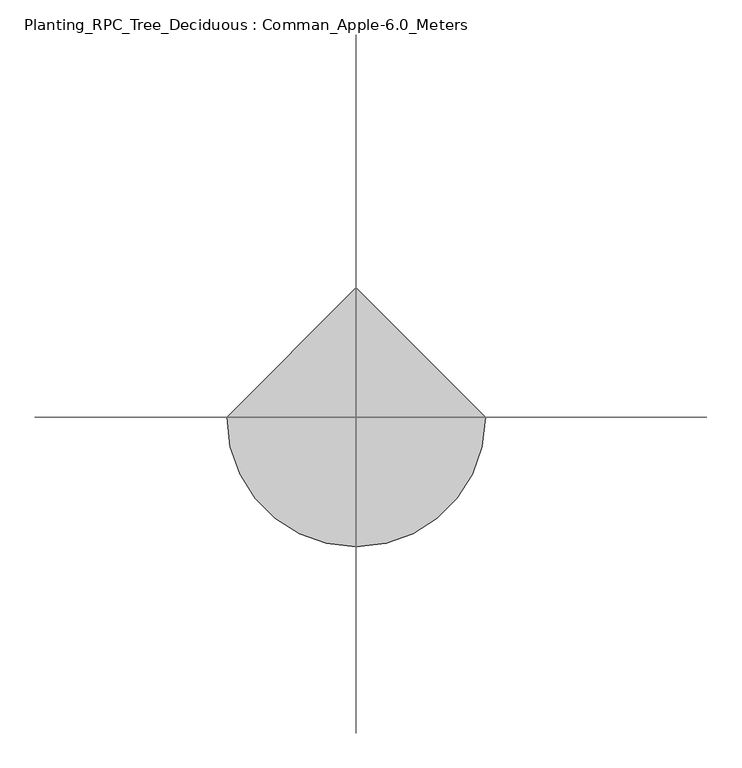
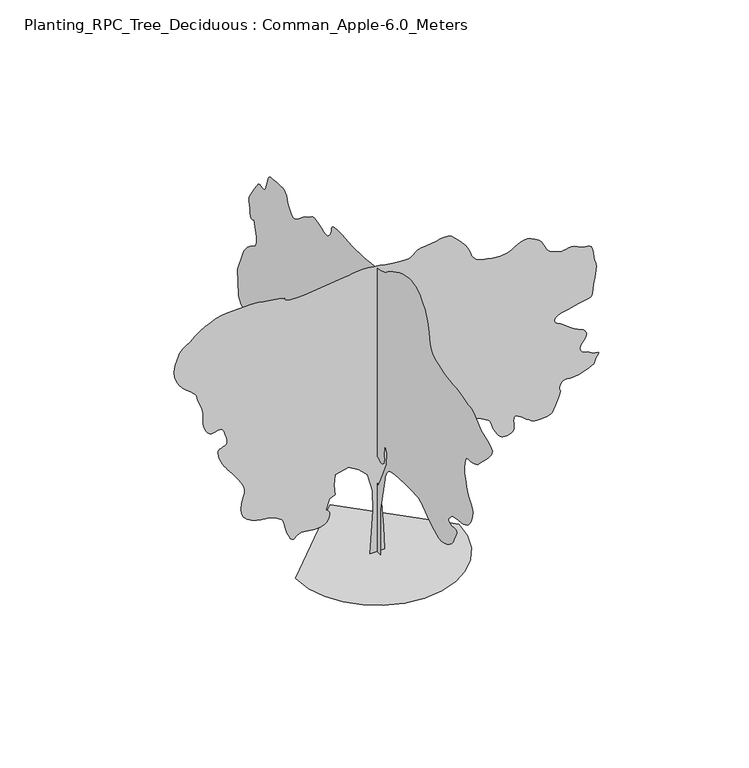
"""IFC4 building model written with IfcOpenShell, lengths in millimetres: geographic element geometry, Planting_RPC_Tree_Deciduous : Comman_Apple-6.0_Meters."""

from ifc_helpers import new_model, si_unit, origin, place, context, project, spatial, triangles, source, transform, mapped, element, save


def planting_rpc_tree_deciduous_comman_apple_6_0_meters_a7a636f8(model_context):
    return source(origin(), model_context, "Body", "Tessellation", [
        triangles([(-6.51e-05, -105.0228319, 0.0074776), (-6.15e-05, 138.9131143, 0.0074703), (-4.84e-05, 99.8833291, 458.6078719), (-3.14e-05, 129.1556067, 1014.7807915), (-1.8e-05, 226.7299288, 1414.8361691), (-8.5e-06, 392.6053236, 1649.0138809), (-1.1e-06, 577.9979682, 1805.1340027), (2.6e-06, 753.6305981, 1844.161417), (3.5e-06, 948.7807503, 1775.8613708), (1.5e-06, 1007.3257959, 1678.2863674), (-4e-06, 890.2357046, 1551.4387321), (-8.4e-06, 929.2657351, 1385.5635372), (-1.44e-05, 1153.685903, 1073.3258371), (-1.47e-05, 1543.9836639, 868.4182137), (-8.5e-06, 2109.9142365, 790.3606236), (7.6e-06, 2451.4244957, 1161.1408985), (2.53e-05, 2802.702182, 1580.7112186), (3.2e-05, 3349.1025513, 1531.9237896), (3.84e-05, 3544.2528488, 1649.0138809), (4.53e-05, 3534.5028625, 1883.1914474), (4.5e-05, 3358.8778267, 1961.2515083), (4.95e-05, 3232.0277206, 2175.9142776), (5.43e-05, 3534.5028625, 2185.6716763), (5.98e-05, 4139.453437, 2068.584201), (6.19e-05, 4208.0283211, 2104.1717091), (6.39e-05, 4273.9283684, 2140.0141434), (6.59e-05, 4334.553447, 2176.3691917), (6.78e-05, 4387.2284294, 2213.4942513), (6.96e-05, 4429.328476, 2251.6417774), (7.12e-05, 4458.2034576, 2291.0693127), (7.26e-05, 4471.2035362, 2332.0343994), (8.79e-05, 4500.4784935, 2829.6522812), (9.79e-05, 4334.6034439, 3249.2275429), (9.86e-05, 4317.5033249, 3282.3275574), (9.94e-05, 4292.2284142, 3321.5527794), (0.0001002, 4260.1033401, 3364.7027618), (0.000101, 4222.5283081, 3409.5526405), (0.0001017, 4180.8532356, 3453.9028404), (0.0001023, 4136.4533295, 3495.527916), (0.0001027, 4090.6782166, 3532.2027122), (0.0001029, 4046.5782921, 3560.9279938), (0.0001029, 4006.7531067, 3582.8278198), (0.000103, 3971.8782005, 3601.8278229), (0.0001031, 3942.6282417, 3621.8527634), (0.0001036, 3919.7031876, 3646.8529816), (0.0001043, 3903.7779968, 3680.7029503), (0.0001056, 3895.5282097, 3727.3530098), (0.0001072, 3894.4779831, 3782.2781456), (0.0001089, 3899.0529945, 3838.2279282), (0.0001108, 3908.3280098, 3895.0532387), (0.0001127, 3921.3530869, 3952.5282188), (0.0001147, 3937.2032822, 4010.528167), (0.0001167, 3954.9280724, 4068.8783844), (0.0001187, 3973.5780968, 4127.4033005), (0.0001184, 3998.5533165, 4107.2783661), (0.0001184, 4022.8532867, 4091.9531387), (0.0001185, 4045.7783409, 4086.1782005), (0.0001191, 4066.6532295, 4094.7532585), (0.0001202, 4084.8032845, 4122.4283134), (0.0001219, 4099.5532562, 4174.003363), (0.0001245, 4110.1781891, 4254.2534065), (0.000127, 4120.6784203, 4333.2285278), (0.0001287, 4132.0283089, 4385.4035408), (0.0001299, 4139.1281662, 4422.2036201), (0.0001309, 4136.8033081, 4455.0786484), (0.0001318, 4120.0031708, 4495.478508), (0.0001331, 4083.5533607, 4554.8286644), (0.0001348, 4022.3783157, 4644.5537109), (0.0001367, 3956.5782623, 4741.1289207), (0.0001382, 3906.9780922, 4815.003772), (0.0001392, 3869.5280525, 4868.5789902), (0.0001398, 3840.0781059, 4904.2041412), (0.0001401, 3814.5529198, 4924.3290756), (0.0001399, 3788.8780334, 4931.3042313), (0.0001393, 3758.9281174, 4927.5038818), (0.0001386, 3727.67799, 4918.0288788), (0.0001379, 3700.2029228, 4909.0788437), (0.0001374, 3675.45298, 4904.7291092), (0.0001372, 3652.4029335, 4909.0788437), (0.0001374, 3630.0528442, 4926.2289597), (0.000138, 3607.3527763, 4960.2792068), (0.0001393, 3583.2777924, 5015.3287537), (0.0001409, 3562.2279144, 5079.6288986), (0.0001424, 3546.3027237, 5137.7538391), (0.0001437, 3531.0527824, 5188.4042358), (0.0001447, 3512.0527794, 5230.1540131), (0.0001452, 3484.8526955, 5261.6794144), (0.0001452, 3445.0278008, 5281.604361), (0.0001446, 3388.1277855, 5288.5295197), (0.0001436, 3319.3276245, 5291.5793335), (0.0001428, 3248.6275795, 5298.5544891), (0.000142, 3178.9774704, 5306.2040222), (0.0001411, 3113.2274139, 5311.3042923), (0.0001402, 3054.3025223, 5310.5793365), (0.0001392, 3005.1273262, 5300.8293503), (0.000138, 2968.5772316, 5278.778952), (0.0001369, 2944.7272339, 5253.1543533), (0.0001361, 2929.602285, 5232.6294434), (0.0001354, 2919.9272942, 5214.0044174), (0.0001347, 2912.4774582, 5194.003894), (0.0001338, 2904.0023941, 5169.4042328), (0.0001326, 2891.2523003, 5136.9288895), (0.000131, 2871.0023735, 5093.3792221), (0.0001292, 2844.6522377, 5045.379245), (0.0001275, 2815.5772682, 5003.1539154), (0.000126, 2783.4271957, 4968.9542587), (0.0001248, 2747.8773308, 4945.0039764), (0.0001238, 2708.5521149, 4933.504097), (0.0001233, 2665.1521477, 4936.7039017), (0.0001232, 2617.3021614, 4956.7788391), (0.0001234, 2569.6771614, 4988.2542435), (0.0001238, 2525.4769524, 5023.3038483), (0.0001243, 2482.1194244, 5060.7288895), (0.0001247, 2437.0593842, 5099.3538574), (0.0001252, 2387.7318718, 5138.0038239), (0.0001254, 2331.5768692, 5175.4288651), (0.0001255, 2266.0343582, 5210.4790512), (0.0001256, 2205.0142456, 5244.5542969), (0.0001259, 2159.0142918, 5277.6040237), (0.0001262, 2120.3541515, 5306.2290207), (0.0001262, 2081.3542065, 5327.0044968), (0.0001258, 2034.3291698, 5336.5044983), (0.0001247, 1971.6040741, 5331.3292328), (0.0001227, 1885.4940685, 5308.0544907), (0.0001205, 1797.391452, 5276.8540695), (0.0001188, 1730.2863911, 5251.9544266), (0.0001175, 1678.8813892, 5236.1042313), (0.0001168, 1637.8888332, 5232.0288986), (0.0001166, 1602.0163136, 5242.4794235), (0.0001169, 1565.9737461, 5270.1544785), (0.0001177, 1524.4687214, 5317.8044769), (0.0001188, 1490.9861721, 5373.8045471), (0.0001201, 1475.2561729, 5423.9793915), (0.0001212, 1466.3511932, 5467.3296524), (0.0001221, 1453.3511147, 5502.8292297), (0.0001225, 1425.3286972, 5529.4543488), (0.0001222, 1371.366148, 5546.1794907), (0.000121, 1280.5334656, 5551.979718), (0.0001195, 1182.4759335, 5550.8792038), (0.0001183, 1108.9958982, 5547.8793869), (0.0001174, 1052.4133781, 5543.5296524), (0.0001165, 1005.0483187, 5538.3293884), (0.0001156, 959.220738, 5532.7791458), (0.0001147, 907.2482563, 5527.4044739), (0.0001136, 841.4482029, 5522.7041794), (0.0001125, 772.3506037, 5519.7043625), (0.0001115, 711.6155754, 5518.9044113), (0.0001107, 653.2705175, 5520.154335), (0.0001099, 591.3404677, 5523.2791443), (0.000109, 519.8504273, 5528.1294296), (0.0001078, 432.8303392, 5534.5046219), (0.0001065, 324.3052774, 5542.2291504), (0.000105, 203.687658, 5552.8796631), (0.0001037, 86.9965703, 5567.6043457), (0.0001026, -21.8426915, 5585.7544006), (0.0001018, -118.9050968, 5606.6292892), (0.0001012, -200.2644113, 5629.5546341), (0.0001011, -261.9952181, 5653.8543137), (0.0001012, -300.1702317, 5678.8295334), (0.0001016, -342.4727732, 5713.0297714), (0.000102, -413.9603428, 5761.2297363), (0.0001023, -506.7854181, 5817.0798157), (0.0001024, -613.0929554, 5874.3298096), (0.0001023, -725.0330704, 5926.6045258), (0.0001019, -834.75319, 5967.6299286), (0.0001011, -934.4057556, 5991.07966), (0.0001, -1022.9033335, 5999.8047089), (9.88e-05, -1104.7484104, 6000.0046967), (9.74e-05, -1180.4459702, 5990.3047073), (9.57e-05, -1250.5110249, 5969.3298248), (9.38e-05, -1315.4560432, 5935.7295502), (9.14e-05, -1375.7936394, 5888.1545471), (8.87e-05, -1432.0336658, 5825.2049011), (8.63e-05, -1478.7161362, 5768.8048553), (8.48e-05, -1512.7687088, 5733.7546692), (8.36e-05, -1538.2837212, 5707.9295013), (8.25e-05, -1559.3636845, 5679.2045105), (8.09e-05, -1580.1012268, 5635.454274), (7.84e-05, -1604.5962433, 5564.5545319), (7.46e-05, -1636.941362, 5454.4042786), (7.05e-05, -1667.1512913, 5330.3292938), (6.7e-05, -1688.656374, 5223.97939), (6.39e-05, -1710.6739254, 5132.8541382), (6.11e-05, -1742.4214062, 5054.3292801), (5.83e-05, -1793.1164223, 4985.8788071), (5.53e-05, -1871.9714928, 4924.9540375), (5.19e-05, -1988.2065491, 4868.9789658), (4.87e-05, -2119.0091755, 4825.5040031), (4.62e-05, -2237.6917568, 4799.6038399), (4.41e-05, -2347.6668755, 4784.9788605), (4.22e-05, -2452.3543808, 4775.3288681), (4.04e-05, -2555.1521759, 4764.2786705), (3.83e-05, -2659.5022018, 4745.5539413), (3.57e-05, -2768.8022163, 4712.8539024), (3.33e-05, -2866.4523605, 4683.5786545), (3.19e-05, -2939.5522591, 4672.2287659), (3.09e-05, -2996.927536, 4668.05373), (2.99e-05, -3047.4773575, 4660.2786232), (2.85e-05, -3100.0773445, 4638.1788094), (2.61e-05, -3163.6025368, 4590.9787834), (2.24e-05, -3246.9276833, 4507.9536186), (1.83e-05, -3354.9527756, 4422.0536293), (1.48e-05, -3474.4277504, 4364.503363), (1.18e-05, -3586.9278603, 4321.8033531), (9.3e-06, -3673.9780701, 4280.47855), (7e-06, -3717.153051, 4227.0283241), (5e-06, -3698.0280556, 4147.9782074), (2.9e-06, -3598.177755, 4029.8281517), (1.1e-06, -3473.4528099, 3906.2781349), (-3e-07, -3385.2276718, 3815.6781418), (-1.3e-06, -3323.4776619, 3751.5279877), (-1.9e-06, -3278.1025246, 3707.3530678), (-2.2e-06, -3239.0275841, 3676.6529068), (-2.3e-06, -3196.2275803, 3652.9528999), (-2.1e-06, -3139.5775497, 3629.777861), (-1.7e-06, -3075.1774109, 3613.37799), (-9e-07, -3016.2275208, 3608.6029907), (-2e-07, -2963.4272552, 3606.7278145), (2e-07, -2917.4774437, 3599.0529922), (2e-07, -2879.0021759, 3576.8528938), (-7e-07, -2848.7272797, 3531.452758), (-2.7e-06, -2827.3521309, 3454.1278267), (-5.1e-06, -2815.7522575, 3369.9277336), (-7e-06, -2813.3521133, 3305.0276253), (-8.6e-06, -2818.6523712, 3252.4026398), (-1.02e-05, -2830.0772552, 3205.052623), (-1.19e-05, -2846.1271477, 3156.0024193), (-1.39e-05, -2865.2274353, 3098.2524559), (-1.64e-05, -2885.9023361, 3024.8022881), (-1.92e-05, -2914.627327, 2946.6774055), (-2.18e-05, -2954.4522217, 2877.5772629), (-2.43e-05, -2998.5524368, 2814.6273262), (-2.67e-05, -3040.0775185, 2754.9021927), (-2.9e-05, -3072.2275909, 2695.5270378), (-3.11e-05, -3088.152491, 2633.6020386), (-3.3e-05, -3081.052343, 2566.2020828), (-3.46e-05, -3060.4274391, 2500.277037), (-3.6e-05, -3039.1022873, 2443.7194427), (-3.71e-05, -3015.2522896, 2395.18694), (-3.79e-05, -2986.9272743, 2353.3118797), (-3.85e-05, -2952.3273514, 2316.7293743), (-3.88e-05, -2909.5023491, 2284.0717747), (-3.89e-05, -2856.6273788, 2253.9743385), (-3.87e-05, -2791.7272705, 2230.5618141), (-3.8e-05, -2717.452153, 2216.0268002), (-3.71e-05, -2638.7520149, 2206.0967377), (-3.62e-05, -2560.5271385, 2196.5117123), (-3.56e-05, -2487.799601, 2182.9993103), (-3.53e-05, -2425.47201, 2161.2942398), (-3.56e-05, -2378.5043827, 2127.129174), (-3.62e-05, -2345.7043499, 2089.8041267), (-3.68e-05, -2322.8042942, 2060.3341232), (-3.73e-05, -2310.1443111, 2037.0066227), (-3.78e-05, -2308.0692924, 2018.1191128), (-3.84e-05, -2316.9168629, 2001.9616688), (-3.92e-05, -2337.029298, 1986.8265461), (-4.01e-05, -2368.7468388, 1971.0090523), (-4.1e-05, -2411.2468609, 1962.5040482), (-4.16e-05, -2459.0394379, 1965.0915356), (-4.21e-05, -2505.4770103, 1970.754126), (-4.27e-05, -2543.876992, 1971.4641117), (-4.34e-05, -2567.6019974, 1959.2041042), (-4.44e-05, -2569.9771431, 1925.949012), (-4.59e-05, -2544.3769615, 1863.6765049), (-4.75e-05, -2509.7520401, 1792.5014889), (-4.89e-05, -2484.8695473, 1735.1513557), (-4.99e-05, -2462.7095627, 1687.5312973), (-5.08e-05, -2436.2819607, 1645.5437439), (-5.14e-05, -2398.5893486, 1605.0912712), (-5.19e-05, -2342.631863, 1562.0787804), (-5.22e-05, -2261.4142914, 1512.4087017), (-5.2e-05, -2169.1316975, 1473.3237328), (-5.1e-05, -2083.5066914, 1461.3762062), (-4.95e-05, -2002.8290577, 1471.4462311), (-4.76e-05, -1925.3965748, 1498.4137711), (-4.53e-05, -1849.4990273, 1537.1587898), (-4.28e-05, -1773.4289612, 1582.5612511), (-4.02e-05, -1695.4838642, 1629.498793), (-3.77e-05, -1622.0062271, 1676.8063705), (-3.54e-05, -1558.0836754, 1724.7963192), (-3.31e-05, -1500.136195, 1770.5689613), (-3.11e-05, -1444.578685, 1811.2214218), (-2.93e-05, -1387.8260445, 1843.8489361), (-2.77e-05, -1326.2960793, 1865.5564774), (-2.64e-05, -1256.4010723, 1873.4340488), (-2.5e-05, -1159.1384045, 1874.2889385), (-2.3e-05, -1027.910804, 1875.4840691), (-2.07e-05, -877.7382116, 1874.971455), (-1.86e-05, -723.6380974, 1870.7039829), (-1.67e-05, -580.6329818, 1860.6339581), (-1.55e-05, -463.7428782, 1842.7115055), (-1.52e-05, -387.9878002, 1814.8914013), (-1.57e-05, -343.2127716, 1776.8839828), (-1.66e-05, -308.1652379, 1730.6863667), (-1.77e-05, -281.2252217, 1677.6614056), (-1.92e-05, -260.7727092, 1619.1738419), (-2.08e-05, -245.1829449, 1556.5887085), (-2.26e-05, -232.8366782, 1491.2736546), (-2.44e-05, -222.1121693, 1424.5935677), (-3.85e-05, -114.7803395, 897.6907001), (-2.01e-05, -26.9632706, 1297.7460777), (-1.3e-05, -173.3248856, 1609.9838505), (-6.5e-06, -300.1727388, 1892.9489914), (2e-07, -319.6852469, 2127.129174), (4.7e-06, -251.3852008, 2244.2167946), (-4e-07, -222.1119331, 2058.8266571), (-1.7e-06, -228.0859325, 2017.1790539), (-3e-06, -232.2679447, 1976.5565334), (-4.1e-06, -232.865183, 1937.9815624), (-5.1e-06, -228.0859325, 1902.4790783), (-5.9e-06, -216.1379155, 1871.0740185), (-6.4e-06, -195.2293988, 1844.788995), (-6.5e-06, -163.5673779, 1824.6489452), (-6.1e-06, -127.1833524, 1819.4714996), (-5.2e-06, -93.5303284, 1831.0189053), (-4.2e-06, -62.949051, 1849.7389835), (-3.3e-06, -35.7820297, 1866.0664753), (-2.9e-06, -12.3698845, 1870.4490566), (-3.1e-06, 6.9458055, 1853.3239391), (-4.3e-06, 21.8237678, 1805.1340027), (-6.1e-06, 32.3777748, 1741.0688725), (-7.7e-06, 39.3472803, 1682.1263947), (-9.3e-06, 43.330036, 1627.4512436), (-1.08e-05, 44.9230347, 1576.1888203), (-1.22e-05, 44.724037, 1527.4862698), (-1.37e-05, 43.330036, 1480.4911732), (-1.51e-05, 41.3385332, 1434.3511116), (137.391859, 0.0003253, 0.0), (-133.3141101, 0.0003334, 0.0), (-73.1573078, 0.0002372, 832.1731876), (-83.1833128, 0.0002433, 1223.1935062), (-183.4456522, 0.0001982, 1574.1087147), (-333.8377625, 0.0002049, 1724.5014244), (-534.3604428, 0.0002126, 1844.8164642), (-785.015601, 0.0002192, 1784.6589443), (-805.0681561, 0.0002168, 1584.1363003), (-785.015601, 0.0002134, 1393.6386257), (-885.278231, 0.0002156, 1343.5060753), (-955.4607931, 0.0002149, 1153.0084007), (-936.3432827, 0.0002675, 1139.8859459), (-918.5407356, 0.0002668, 1125.3558735), (-903.3707314, 0.0002661, 1108.0233559), (-892.1456898, 0.0002654, 1086.4808481), (-886.1831903, 0.0002648, 1059.3258196), (-886.7981964, 0.0002643, 1025.1533415), (-895.3032005, 0.0002639, 982.565752), (-913.9532249, 0.0002639, 940.0632591), (-942.5982788, 0.0002642, 906.5057144), (-978.963283, 0.0002649, 881.0181713), (-1020.7633478, 0.0002659, 862.7181982), (-1065.71838, 0.0002671, 850.7331739), (-1111.553373, 0.0002683, 844.1856812), (-1155.9834372, 0.0002696, 842.1981571), (-1199.4784567, 0.000271, 844.8881819), (-1243.6759769, 0.0002724, 851.4356747), (-1288.0485592, 0.0002738, 859.5631582), (-1332.0685467, 0.0002752, 866.9856703), (-1375.2135876, 0.0002766, 871.4282043), (-1416.9560978, 0.0002778, 870.610667), (-1456.7686386, 0.0002789, 862.2507122), (-1490.9986713, 0.0002796, 844.3906832), (-1518.2137253, 0.0002801, 821.2681847), (-1541.2187164, 0.0002805, 799.9006662), (-1562.8187061, 0.0002809, 787.3031067), (-1585.8236973, 0.0002817, 790.4881594), (-1613.0387512, 0.0002829, 816.475672), (-1647.2663132, 0.0002313, 872.2782251), (-1679.7413658, 0.0002334, 944.3882858), (-1702.0463997, 0.0002351, 1013.3457773), (-1717.508828, 0.0002365, 1077.2133905), (-1729.4639122, 0.0002377, 1134.0684231), (-1741.2438618, 0.0002387, 1181.9784348), (-1756.1814674, 0.0002397, 1219.0134562), (-1777.6064678, 0.0002407, 1243.2460613), (-1804.2939377, 0.0002418, 1262.5659576), (-1833.963929, 0.000243, 1284.8709915), (-1868.368951, 0.0002444, 1308.2261066), (-1909.2639839, 0.000246, 1330.7035137), (-1958.3990662, 0.0002477, 1350.3761501), (-2017.5341194, 0.0002497, 1365.3136105), (-2088.4191822, 0.0002519, 1373.5860706), (-2170.7616852, 0.0002011, 1382.5010788), (-2258.5417923, 0.000204, 1401.9385551), (-2344.9193687, 0.0002071, 1433.8310852), (-2423.054425, 0.0002101, 1480.1036968), (-2486.1043556, 0.0002129, 1542.6862141), (-2527.2271362, 0.0002153, 1623.5087517), (-2539.6019623, 0.0002172, 1724.5014244), (-2528.5270569, 0.0002183, 1822.2489464), (-2508.6771057, 0.0002189, 1897.5490013), (-2487.2420769, 0.0002192, 1958.6416386), (-2471.4293793, 0.0001661, 2013.7690876), (-2468.4170631, 0.0001669, 2071.1791008), (-2485.3994568, 0.0001684, 2139.1117275), (-2529.5769928, 0.000171, 2225.8093426), (-2588.3771828, 0.0001741, 2318.6767845), (-2644.0269836, 0.000177, 2400.3194756), (-2695.8270195, 0.0001796, 2471.7869156), (-2743.0773331, 0.000182, 2534.1270058), (-2785.0520966, 0.0001306, 2588.4271797), (-2821.0522247, 0.0001324, 2635.6772026), (-2850.4021774, 0.0001339, 2676.9770073), (-2878.5522034, 0.0001354, 2723.8270546), (-2908.6274025, 0.0001372, 2782.7522369), (-2936.4274498, 0.000139, 2847.4523575), (-2957.7523109, 0.0001406, 2911.6522179), (-2968.3522453, 0.0001418, 2969.0024963), (-2964.0525078, 0.0001423, 3013.2024147), (-2940.6524826, 0.000142, 3037.927359), (-2905.0023331, 0.0001411, 3050.052491), (-2869.2021927, 0.0001402, 3062.5523094), (-2836.72714, 0.0001395, 3078.1775185), (-2811.1022507, 0.000139, 3099.7773628), (-2795.8023125, 0.000139, 3130.1525436), (-2794.3771088, 0.0001396, 3172.1025993), (-2810.3022995, 0.0001409, 3228.4276497), (-2831.7271545, 8.9e-05, 3286.3526024), (-2846.6774048, 9.02e-05, 3332.2027107), (-2858.4522675, 9.1e-05, 3367.3276016), (-2870.4024101, 9.18e-05, 3393.1777679), (-2885.8523392, 9.25e-05, 3411.1278351), (-2908.17743, 9.33e-05, 3422.5777176), (-2940.6524826, 9.44e-05, 3428.9526192), (-2978.7524826, 9.55e-05, 3427.0527351), (-3016.0025345, 9.65e-05, 3417.4277412), (-3052.7023293, 9.74e-05, 3407.1277885), (-3089.2524239, 9.85e-05, 3403.1027435), (-3125.9775078, 9.97e-05, 3412.4277557), (-3163.2025612, 0.0001012, 3442.1026886), (-3201.3275597, 0.0001032, 3499.1276962), (-3229.5025841, 0.0001051, 3569.6277534), (-3241.3777313, 0.0001065, 3637.1529922), (-3243.9525742, 0.0001076, 3704.8529297), (-3244.2275574, 0.0001086, 3775.9029533), (-3249.2525414, 5.65e-05, 3853.4031647), (-3266.0276802, 5.83e-05, 3940.5780762), (-3301.5775452, 6.09e-05, 4040.5533691), (-3337.877655, 6.33e-05, 4130.928376), (-3357.5276184, 6.48e-05, 4192.7283829), (-3368.4028267, 6.58e-05, 4234.1784691), (-3378.4027977, 6.65e-05, 4263.5284218), (-3395.4276306, 6.74e-05, 4289.0033203), (-3427.3277184, 6.88e-05, 4318.8785316), (-3482.0528664, 7.1e-05, 4361.3785538), (-3552.8529053, 2.06e-05, 4417.8785934), (-3623.6529442, 2.37e-05, 4484.3786041), (-3688.3030678, 2.68e-05, 4561.0535751), (-3740.6780685, 2.96e-05, 4648.0787865), (-3774.6530296, 3.21e-05, 4745.6289368), (-3784.0780357, 3.4e-05, 4853.8540169), (-3762.7778824, 3.51e-05, 4972.9790131), (-3729.8778557, -1.77e-05, 5076.7040771), (-3704.502951, -1.74e-05, 5145.8539261), (-3680.7029503, -1.74e-05, 5191.3290573), (-3652.5279259, -1.78e-05, 5224.0043884), (-3614.0029518, -1.85e-05, 5254.7792542), (-3559.1778099, -1.95e-05, 5294.454158), (-3482.0528664, -2.09e-05, 5353.9790131), (-3391.1775993, -2.26e-05, 5424.8793365), (-3298.9027084, -2.44e-05, 5490.3794083), (-3205.0276245, -2.63e-05, 5548.6543396), (-3109.4273552, -2.84e-05, 5598.0042343), (-3011.8774956, -3.07e-05, 5636.6297836), (-2912.2274734, -3.33e-05, 5662.8293472), (-2810.3022995, -3.62e-05, 5674.8047791), (-2339.0719059, -5.01e-05, 5684.8297485), (-2273.3618179, -5.21e-05, 5682.2043274), (-2197.6542297, -5.44e-05, 5674.854776), (-2113.614156, -3.7e-06, 5663.5293045), (-2022.9115528, -6.6e-06, 5649.0546066), (-1927.2115803, -9.7e-06, 5632.2294708), (-1828.1764915, -1.3e-05, 5613.8044327), (-1727.4763882, -1.63e-05, 5594.6044418), (-1724.3188774, -1.66e-05, 5575.4544479), (-1715.1112999, -1.72e-05, 5557.4543839), (-1693.8014088, -1.8e-05, 5541.7291809), (-1654.3413174, -1.94e-05, 5529.4293503), (-1590.6763081, -2.14e-05, 5521.6792419), (-1496.7561687, -2.42e-05, 5519.6293671), (-1366.5335941, -2.81e-05, 5524.4296555), (-604.5454757, -4.94e-05, 5614.6543808), (-529.8304141, -5.15e-05, 5621.554541), (-464.7628741, 1e-07, 5631.7794983), (-403.0278342, -1.6e-06, 5642.554422), (-338.3102729, -3.4e-06, 5651.0294861), (-264.297712, -5.6e-06, 5654.4042801), (-174.6758932, -8.3e-06, 5649.9045547), (-63.1312982, -1.19e-05, 5634.7043198), (53.8502923, -1.57e-05, 5614.4793915), (156.9766284, -1.9e-05, 5596.879303), (248.3524462, -2.19e-05, 5582.1046234), (330.0827591, -2.45e-05, 5570.2791824), (404.2703093, -2.69e-05, 5561.6297104), (473.0203643, -2.9e-05, 5556.304454), (538.4379192, -3.1e-05, 5554.5045639), (593.7429737, -3.25e-05, 5562.8296371), (635.895488, -3.35e-05, 5584.3044891), (672.6080727, -3.41e-05, 5613.6794403), (711.6030762, -3.48e-05, 5645.7042297), (760.5931091, -3.58e-05, 5675.0797623), (827.2981945, -3.75e-05, 5696.5546143), (919.4332684, -4.01e-05, 5704.904686), (1019.3733164, -4.3e-05, 5711.6048584), (1106.3358862, -4.54e-05, 5726.7545151), (1183.3009558, -4.74e-05, 5742.7796997), (1253.2485031, -4.94e-05, 5752.1297104), (1319.1659912, -5.14e-05, 5747.279425), (1384.0286018, -5.37e-05, 5720.6793045), (1450.8211819, -3.2e-06, 5664.7798096), (1514.7787605, -6.1e-06, 5597.4042709), (1569.6162563, -8.6e-06, 5539.5043167), (1616.0337719, -1.07e-05, 5488.254538), (1654.7363514, -1.26e-05, 5440.8795227), (1686.421336, -1.42e-05, 5394.5544434), (1711.7939152, -1.57e-05, 5346.4544724), (1731.5539009, -1.7e-05, 5293.8291962), (1749.3263626, -1.84e-05, 5241.0039322), (1770.606459, -1.97e-05, 5194.1538849), (1798.9013889, -2.12e-05, 5153.0790665), (1837.7189323, 3.06e-05, 5117.6039063), (1890.5690495, 2.85e-05, 5087.6039932), (1960.9566135, 2.61e-05, 5062.8287613), (2052.3915848, 2.3e-05, 5043.1537994), (2147.2741653, 2e-05, 5028.9540848), (2227.0742363, 1.75e-05, 5020.3540283), (2293.8969017, 1.55e-05, 5016.8542419), (2349.8443588, 1.38e-05, 5017.9041779), (2397.0244732, 1.25e-05, 5023.0038666), (2437.5369713, 1.14e-05, 5031.5789246), (2473.4920441, 1.05e-05, 5043.1537994), (2512.0269012, 9.7e-06, 5063.479303), (2558.2519867, 8.7e-06, 5093.9791855), (2611.3522339, 7.6e-06, 5127.6038773), (2670.3771194, 6.3e-06, 5157.4043839), (2734.5272736, 4.7e-06, 5176.304393), (2802.8521729, 2.7e-06, 5177.3293304), (2874.5271584, 2e-07, 5153.4540436), (2937.3023964, -2.2e-06, 5120.2293274), (2982.5272522, -3.9e-06, 5095.0541199), (3014.7523201, -5.2e-06, 5073.7292587), (3038.5773193, -6.2e-06, 5052.0788361), (3058.5525536, -7.2e-06, 5025.854274), (3079.2024559, -8.3e-06, 4990.8790833), (3105.1276176, -9.8e-06, 4942.9041046), (3132.7273865, 4.2e-05, 4892.8036743), (3157.7026062, 4.07e-05, 4852.7037964), (3183.5274834, 3.94e-05, 4820.3037392), (3213.7526733, 3.81e-05, 4793.3539307), (3251.8776718, 3.66e-05, 4769.5539299), (3301.4025558, 3.48e-05, 4746.6538742), (3365.8276932, 3.25e-05, 4722.3289055), (3431.1277771, 3.03e-05, 4707.5036476), (3484.3277275, 2.88e-05, 4709.3538254), (3530.502816, 2.76e-05, 4719.9537598), (3574.7527313, 2.64e-05, 4731.4539299), (3622.1780342, 2.51e-05, 4735.9286568), (3677.8278351, 2.33e-05, 4725.4787132), (3746.8029854, 2.07e-05, 4692.2537064), (3818.1279922, 1.81e-05, 4658.4537346), (3877.8781242, 1.61e-05, 4644.1287369), (3926.7530479, 1.45e-05, 4638.053817), (3965.453302, 1.32e-05, 4629.003788), (3994.7032608, 1.2e-05, 4605.7287552), (4015.1531754, 6.41e-05, 4557.0285301), (4027.5532906, 6.24e-05, 4471.6785072), (4039.2031609, 6.08e-05, 4384.4785973), (4054.5533867, 5.95e-05, 4327.8035683), (4069.9033218, 5.84e-05, 4286.7284592), (4081.5781906, 5.75e-05, 4246.3533073), (4085.8532204, 5.65e-05, 4191.7784409), (4079.1033417, 5.55e-05, 4108.1033157), (4057.628199, 5.42e-05, 3980.3782631), (4035.5280945, 0.0001063, 3847.1779633), (4024.4781876, 0.0001052, 3752.0279572), (4017.103347, 0.0001045, 3687.5778214), (4006.0531494, 0.0001042, 3646.453006), (3983.9530449, 0.0001045, 3621.2777985), (3943.4531914, 0.0001054, 3604.7279366), (3877.1531685, 0.0001072, 3589.3780014), (3783.9280449, 0.0001097, 3571.4279343), (3675.2779907, 0.0001126, 3551.3777046), (3562.7778809, 0.0001156, 3528.3279488), (3457.9778824, 0.0001183, 3501.452845), (3372.477578, 0.0001204, 3469.8277405), (3317.8527145, 0.0001215, 3432.5776886), (3305.6525871, 0.0001212, 3388.8527412), (3318.4276794, 0.0001203, 3351.9776665), (3332.9526649, 0.0001195, 3330.9027901), (3352.2276512, 0.0001188, 3318.0777008), (3379.2027489, 0.0001178, 3305.9525688), (3416.8777748, 0.0001164, 3286.9775642), (3468.2528366, 0.0001143, 3253.627565), (3536.2527557, 0.0001115, 3198.3524506), (3611.5028137, 0.0001084, 3139.7525391), (3681.477903, 0.0001057, 3097.8024834), (3744.6281181, 0.0001033, 3067.0773239), (3799.3529755, 0.0001547, 3042.1273933), (3844.053154, 0.000153, 3017.5524399), (3877.2031654, 0.0001516, 2987.877507), (3897.2031075, 0.0001504, 2947.702343), (3897.9280632, 0.0001497, 2900.4773186), (3879.7280113, 0.0001495, 2853.6272713), (3850.6530418, 0.0001497, 2807.4771812), (3818.7529541, 0.00015, 2762.3773178), (3792.1281258, 0.0001501, 2718.6770782), (3778.8280655, 0.0001499, 2676.7270226), (3786.9281525, 0.0001491, 2636.8771294), (3809.6279297, 0.0001479, 2605.4770111), (3834.8031372, 0.0001469, 2585.8520462), (3862.4281952, 0.0001459, 2573.7522034), (3892.5031036, 0.0001448, 2564.9771576), (3925.0281532, 0.0001437, 2555.3271652), (3960.0280518, 0.0001425, 2540.6019012), (3997.4780914, 0.000141, 2516.5769142), (4036.1783455, 0.0001395, 2494.674472), (4072.603157, 0.0001383, 2485.0593613), (4103.2283226, 0.0001373, 2481.5793411), (4124.5531837, 0.0001366, 2478.1019371), (4133.1032433, 0.0001362, 2468.4845009), (4125.3284271, 0.0001895, 2446.5919418), (4097.7283676, 0.0001897, 2406.2819023), (4070.2033035, 0.0001899, 2361.9969601), (4057.9281807, 0.0001898, 2329.461882), (4050.3783508, 0.0001896, 2304.4693668), (4037.0532921, 0.0001897, 2282.8093517), (4007.403067, 0.0001903, 2260.2742447), (3950.9280258, 0.0001915, 2232.649332), (3857.1032295, 0.0001938, 2195.731818), (3751.1030136, 0.0001965, 2165.9741867), (3663.5278358, 0.000199, 2156.5616798), (3591.9278458, 0.0002011, 2158.3742146), (3533.8029053, 0.0002029, 2162.291708), (3486.7528702, 0.0002043, 2159.1942226), (3448.2778931, 0.0002051, 2139.9592049), (3415.9528313, 0.0002054, 2095.4691879), (3396.9028313, 0.0002053, 2048.9641777), (3394.8526657, 0.000205, 2022.9766651), (3402.2777939, 0.0002045, 2007.3391022), (3411.6278046, 0.000204, 1991.8765285), (3415.3778664, 0.0002035, 1966.4166), (3405.9528603, 0.0002031, 1920.7865364), (3375.8526627, 0.0002029, 1844.8164642), (3339.8025375, 0.0002027, 1759.2289558), (3313.4026955, 0.0002024, 1690.476321), (3290.3526489, 0.0002023, 1636.9838013), (3264.3024948, 0.0002025, 1597.1712605), (3228.9526176, 0.0002032, 1569.4613239), (3178.0025299, 0.0002044, 1552.2737103), (3105.1276176, 0.0002065, 1544.0311901), (3032.1274223, 0.0002086, 1540.6111954), (2980.1523972, 0.0002101, 1539.996262), (2942.0273987, 0.0002113, 1543.7687061), (2910.5772835, 0.0002124, 1553.5012516), (2878.6022003, 0.0002136, 1570.7762146), (2838.902298, 0.0002152, 1597.1712605), (2784.3021423, 0.0002174, 1634.2663799), (2725.2272598, 0.0002198, 1675.6263554), (2676.327047, 0.0002218, 1712.2539162), (2636.7271385, 0.0002234, 1741.8638821), (2605.5270081, 0.0002246, 1762.1813919), (2581.8769981, 0.0002254, 1770.9214108), (2564.9021622, 0.0002259, 1765.8038452), (2553.7019737, 0.0002259, 1744.5538342), (2547.3770691, 0.0002257, 1717.2514309), (2544.9269279, 0.0002254, 1694.3364052), (2545.2769066, 0.0002251, 1674.0488354), (2547.3770691, 0.0002247, 1654.6388283), (2550.2018967, 0.0002244, 1634.3538746), (2552.6520378, 0.0002239, 1611.4362328), (2553.7019737, 0.0002235, 1584.1363003), (2552.2770607, 0.0002231, 1554.2312943), (2547.1520828, 0.0002228, 1525.3811657), (2537.1271133, 0.0002227, 1498.6361412), (2520.9519379, 0.0002229, 1475.0461567), (2497.4295364, 0.0002233, 1455.666235), (2465.3044624, 0.000224, 1441.5461666), (2423.3594936, 0.0002251, 1433.7435905), (2380.6244568, 0.0002264, 1432.0761051), (2345.4293667, 0.0002275, 1436.3736626), (2315.4968914, 0.0002286, 1447.6861988), (2288.5467922, 0.0002297, 1467.0661205), (2262.2967957, 0.0002309, 1495.5661251), (2234.4692791, 0.0002323, 1534.2387646), (2202.7842945, 0.000234, 1584.1363003), (2173.4642818, 0.0002356, 1638.6213467), (2152.3892601, 0.0001837, 1689.7763638), (2136.7516972, 0.0001848, 1736.7213181), (2123.7442062, 0.0001858, 1778.5789375), (2110.561726, 0.0001868, 1814.4739849), (2094.3967243, 0.0001877, 1843.5290428), (2072.4441399, 0.0001886, 1864.8690193), (2041.9866966, 0.0001898, 1883.516573), (2003.1091278, 0.0001913, 1904.796524), (1957.2165802, 0.000193, 1928.2690739), (1905.7115845, 0.0001949, 1953.4966038), (1849.996526, 0.000197, 1980.0365536), (1791.4764061, 0.0001991, 2007.4565369), (1731.5539009, 0.0002013, 2035.3141388), (1390.663662, 0.0002115, 2035.3141388), (1200.1659874, 0.0002139, 1814.7364689), (1195.6959841, 0.0002136, 1784.6589443), (1190.1709579, 0.0002133, 1754.578949), (1182.5409731, 0.0002131, 1724.5014244), (1171.7559483, 0.0002129, 1694.4238998), (1156.7583899, 0.0002129, 1664.3437592), (1136.5033762, 0.0002131, 1634.2663799), (1109.9308702, 0.0002134, 1604.1888554), (1086.2834038, 0.0002138, 1578.7562508), (1071.7558748, 0.0002139, 1561.5687824), (1060.7358353, 0.0002141, 1551.0461689), (1047.610837, 0.0002144, 1545.6087101), (1026.7682865, 0.000215, 1543.6787407), (992.5982792, 0.000216, 1543.6787407), (939.4857508, 0.0002176, 1544.0311901), (873.0156801, 0.0002196, 1546.8661915), (804.2656614, 0.0002218, 1554.4362236), (735.8656214, 0.000224, 1565.3387558), (670.4455593, 0.0002262, 1578.1712574), (610.6404888, 0.0002281, 1591.5313431), (559.0754313, 0.0002299, 1604.0112499), (518.3879076, 0.0002312, 1614.2138248), (483.4279049, 0.0002324, 1624.5613037), (447.4153502, 0.0002337, 1638.0662933), (410.5253417, 0.000235, 1654.201355), (372.9353033, 0.0002364, 1672.4413754), (334.8177535, 0.0001845, 1692.2589157), (296.3502432, 0.0001859, 1713.1313335), (257.7052002, 0.0001874, 1734.5288647), (77.2350658, 0.0002405, 1353.5335155), (67.2090517, 0.0002365, 1062.7733562), (117.3398399, 0.0002792, 451.1778749), (-1522.7162121, 1.1e-06, 0.0098235), (-1482.4612564, -348.9052657, 0.0098339), (-1367.8136032, -669.3205553, 0.0098435), (-1187.9534334, -952.0632534, 0.0098519), (-952.0632534, -1187.9534334, 0.0098589), (-669.3205553, -1367.8136032, 0.0098643), (-348.9052657, -1482.4612564, 0.0098677), (6.66e-05, -1522.7162121, 0.0098689), (348.9052657, -1482.4612564, 0.0098677), (669.3205553, -1367.8136032, 0.0098643), (952.0632534, -1187.9534334, 0.0098589), (1187.9534334, -952.0632534, 0.0098519), (1367.8136032, -669.3205553, 0.0098435), (1482.4612564, -348.9052657, 0.0098339), (1522.7162121, 0.0001238, 0.0098235), (-0.0001997, 1522.7162121, 0.0097782)], [[300, 1, 301], [299, 300, 301], [299, 301, 302], [298, 299, 302], [297, 298, 302], [296, 297, 302], [296, 302, 303], [295, 296, 303], [294, 295, 303], [293, 294, 303], [292, 293, 303], [1, 2, 3], [301, 1, 3], [301, 3, 4], [301, 4, 5], [327, 301, 5], [326, 327, 5], [326, 5, 6], [325, 326, 6], [324, 325, 6], [323, 324, 6], [322, 323, 6], [321, 322, 6], [320, 321, 6], [19, 20, 21], [18, 19, 21], [17, 18, 21], [17, 21, 22], [320, 6, 7], [319, 320, 7], [291, 292, 303], [291, 303, 304], [290, 291, 304], [261, 262, 263], [260, 261, 263], [260, 263, 264], [259, 260, 264], [259, 264, 265], [258, 259, 265], [10, 11, 12], [14, 15, 16], [258, 265, 266], [257, 258, 266], [205, 206, 207], [204, 205, 207], [204, 207, 208], [203, 204, 208], [203, 208, 209], [202, 203, 209], [202, 209, 210], [257, 266, 267], [10, 12, 13], [257, 267, 268], [257, 268, 269], [256, 257, 269], [256, 269, 270], [256, 270, 271], [255, 256, 271], [255, 271, 272], [255, 272, 273], [255, 273, 274], [255, 274, 275], [255, 275, 276], [255, 276, 277], [254, 255, 277], [254, 277, 278], [254, 278, 279], [254, 279, 280], [253, 254, 280], [253, 280, 281], [253, 281, 282], [289, 290, 304], [10, 13, 14], [10, 14, 16], [10, 16, 17], [10, 17, 22], [9, 10, 22], [201, 202, 210], [201, 210, 211], [201, 211, 212], [201, 212, 213], [201, 213, 214], [201, 214, 215], [201, 215, 216], [201, 216, 217], [201, 217, 218], [201, 218, 219], [200, 201, 219], [199, 200, 219], [198, 199, 219], [197, 198, 219], [196, 197, 219], [195, 196, 219], [194, 195, 219], [194, 219, 220], [193, 194, 220], [192, 193, 220], [191, 192, 220], [190, 191, 220], [189, 190, 220], [189, 220, 221], [188, 189, 221], [252, 253, 282], [252, 282, 283], [188, 221, 222], [187, 188, 222], [251, 252, 283], [187, 222, 223], [23, 24, 25], [318, 319, 7], [56, 57, 58], [56, 58, 59], [55, 56, 59], [55, 59, 60], [54, 55, 60], [54, 60, 61], [54, 61, 62], [23, 25, 26], [186, 187, 223], [23, 26, 27], [23, 27, 28], [23, 28, 29], [23, 29, 30], [23, 30, 31], [23, 31, 32], [23, 32, 33], [23, 33, 34], [23, 34, 35], [23, 35, 36], [23, 36, 37], [23, 37, 38], [23, 38, 39], [23, 39, 40], [23, 40, 41], [23, 41, 42], [23, 42, 43], [23, 43, 44], [22, 23, 44], [22, 44, 45], [9, 22, 45], [9, 45, 46], [9, 46, 47], [9, 47, 48], [8, 9, 48], [8, 48, 49], [8, 49, 50], [8, 50, 51], [8, 51, 52], [8, 52, 53], [8, 53, 54], [250, 251, 283], [250, 283, 284], [288, 289, 304], [288, 304, 305], [186, 223, 224], [287, 288, 305], [313, 314, 315], [312, 313, 315], [311, 312, 315], [310, 311, 315], [310, 315, 316], [309, 310, 316], [308, 309, 316], [308, 316, 317], [307, 308, 317], [306, 307, 317], [306, 317, 318], [305, 306, 318], [305, 318, 7], [305, 7, 8], [305, 8, 54], [305, 54, 62], [305, 62, 63], [305, 63, 64], [305, 64, 65], [305, 65, 66], [305, 66, 67], [305, 67, 68], [305, 68, 69], [305, 69, 70], [305, 70, 71], [305, 71, 72], [305, 72, 73], [305, 73, 74], [305, 74, 75], [305, 75, 76], [305, 76, 77], [305, 77, 78], [305, 78, 79], [305, 79, 80], [305, 80, 81], [305, 81, 82], [305, 82, 83], [305, 83, 84], [305, 84, 85], [305, 85, 86], [305, 86, 87], [305, 87, 88], [305, 88, 89], [305, 89, 90], [305, 90, 91], [305, 91, 92], [134, 135, 136], [134, 136, 137], [133, 134, 137], [133, 137, 138], [132, 133, 138], [132, 138, 139], [132, 139, 140], [131, 132, 140], [131, 140, 141], [131, 141, 142], [131, 142, 143], [130, 131, 143], [130, 143, 144], [130, 144, 145], [286, 287, 305], [186, 224, 225], [185, 186, 225], [249, 250, 284], [130, 145, 146], [285, 286, 305], [249, 284, 285], [249, 285, 305], [248, 249, 305], [234, 235, 236], [233, 234, 236], [233, 236, 237], [232, 233, 237], [232, 237, 238], [232, 238, 239], [232, 239, 240], [232, 240, 241], [232, 241, 242], [232, 242, 243], [232, 243, 244], [232, 244, 245], [231, 232, 245], [231, 245, 246], [231, 246, 247], [230, 231, 247], [230, 247, 248], [230, 248, 305], [229, 230, 305], [228, 229, 305], [227, 228, 305], [226, 227, 305], [225, 226, 305], [185, 225, 305], [184, 185, 305], [183, 184, 305], [182, 183, 305], [181, 182, 305], [180, 181, 305], [179, 180, 305], [178, 179, 305], [177, 178, 305], [176, 177, 305], [175, 176, 305], [174, 175, 305], [173, 174, 305], [172, 173, 305], [171, 172, 305], [170, 171, 305], [169, 170, 305], [168, 169, 305], [167, 168, 305], [166, 167, 305], [165, 166, 305], [164, 165, 305], [163, 164, 305], [162, 163, 305], [161, 162, 305], [160, 161, 305], [159, 160, 305], [158, 159, 305], [157, 158, 305], [156, 157, 305], [155, 156, 305], [154, 155, 305], [153, 154, 305], [152, 153, 305], [151, 152, 305], [150, 151, 305], [149, 150, 305], [148, 149, 305], [147, 148, 305], [146, 147, 305], [130, 146, 305], [129, 130, 305], [128, 129, 305], [127, 128, 305], [126, 127, 305], [125, 126, 305], [124, 125, 305], [123, 124, 305], [122, 123, 305], [121, 122, 305], [120, 121, 305], [119, 120, 305], [118, 119, 305], [117, 118, 305], [116, 117, 305], [115, 116, 305], [114, 115, 305], [113, 114, 305], [112, 113, 305], [111, 112, 305], [110, 111, 305], [109, 110, 305], [108, 109, 305], [107, 108, 305], [94, 95, 96], [94, 96, 97], [93, 94, 97], [93, 97, 98], [93, 98, 99], [93, 99, 100], [93, 100, 101], [92, 93, 101], [92, 101, 102], [92, 102, 103], [92, 103, 104], [92, 104, 105], [106, 107, 305], [106, 305, 92], [106, 92, 105], [328, 329, 330], [731, 328, 330], [730, 731, 330], [730, 330, 331], [729, 730, 331], [729, 331, 332], [728, 729, 332], [472, 473, 474], [336, 337, 338], [728, 332, 333], [618, 619, 620], [617, 618, 620], [617, 620, 621], [616, 617, 621], [615, 616, 621], [615, 621, 622], [614, 615, 622], [614, 622, 623], [472, 474, 475], [613, 614, 623], [612, 613, 623], [612, 623, 624], [612, 624, 625], [612, 625, 626], [612, 626, 627], [612, 627, 628], [611, 612, 628], [610, 611, 628], [610, 628, 629], [609, 610, 629], [609, 629, 630], [608, 609, 630], [608, 630, 631], [608, 631, 632], [607, 608, 632], [607, 632, 633], [606, 607, 633], [363, 364, 365], [363, 365, 366], [362, 363, 366], [362, 366, 367], [361, 362, 367], [361, 367, 368], [360, 361, 368], [360, 368, 369], [360, 369, 370], [359, 360, 370], [359, 370, 371], [358, 359, 371], [358, 371, 372], [407, 408, 409], [407, 409, 410], [406, 407, 410], [406, 410, 411], [405, 406, 411], [405, 411, 412], [404, 405, 412], [403, 404, 412], [403, 412, 413], [402, 403, 413], [401, 402, 413], [400, 401, 413], [399, 400, 413], [357, 358, 372], [606, 633, 634], [399, 413, 414], [398, 399, 414], [728, 333, 334], [357, 372, 373], [356, 357, 373], [562, 563, 564], [561, 562, 564], [561, 564, 565], [560, 561, 565], [559, 560, 565], [559, 565, 566], [397, 398, 414], [355, 356, 373], [354, 355, 373], [353, 354, 373], [352, 353, 373], [351, 352, 373], [350, 351, 373], [349, 350, 373], [348, 349, 373], [347, 348, 373], [346, 347, 373], [345, 346, 373], [344, 345, 373], [343, 344, 373], [342, 343, 373], [341, 342, 373], [340, 341, 373], [339, 340, 373], [338, 339, 373], [336, 338, 373], [336, 373, 374], [335, 336, 374], [335, 374, 375], [335, 375, 376], [335, 376, 377], [335, 377, 378], [335, 378, 379], [335, 379, 380], [576, 577, 578], [575, 576, 578], [575, 578, 579], [574, 575, 579], [574, 579, 580], [573, 574, 580], [573, 580, 581], [572, 573, 581], [572, 581, 582], [571, 572, 582], [570, 571, 582], [569, 570, 582], [568, 569, 582], [567, 568, 582], [566, 567, 582], [559, 566, 582], [558, 559, 582], [557, 558, 582], [556, 557, 582], [555, 556, 582], [554, 555, 582], [553, 554, 582], [552, 553, 582], [552, 582, 583], [551, 552, 583], [551, 583, 584], [550, 551, 584], [549, 550, 584], [549, 584, 585], [548, 549, 585], [547, 548, 585], [546, 547, 585], [599, 600, 601], [598, 599, 601], [598, 601, 602], [597, 598, 602], [597, 602, 603], [596, 597, 603], [596, 603, 604], [595, 596, 604], [595, 604, 605], [594, 595, 605], [594, 605, 606], [594, 606, 634], [593, 594, 634], [592, 593, 634], [591, 592, 634], [590, 591, 634], [589, 590, 634], [588, 589, 634], [588, 634, 635], [587, 588, 635], [587, 635, 636], [545, 546, 585], [335, 380, 381], [427, 428, 429], [426, 427, 429], [426, 429, 430], [425, 426, 430], [425, 430, 431], [424, 425, 431], [424, 431, 432], [424, 432, 433], [423, 424, 433], [423, 433, 434], [422, 423, 434], [422, 434, 435], [422, 435, 436], [421, 422, 436], [335, 381, 382], [335, 382, 383], [335, 383, 384], [335, 384, 385], [335, 385, 386], [335, 386, 387], [335, 387, 388], [335, 388, 389], [335, 389, 390], [335, 390, 391], [335, 391, 392], [335, 392, 393], [335, 393, 394], [335, 394, 395], [335, 395, 396], [335, 396, 397], [335, 397, 414], [335, 414, 415], [334, 335, 415], [334, 415, 416], [334, 416, 417], [334, 417, 418], [334, 418, 419], [334, 419, 420], [728, 334, 420], [638, 639, 640], [638, 640, 641], [638, 641, 642], [637, 638, 642], [545, 585, 586], [544, 545, 586], [728, 420, 421], [728, 421, 436], [728, 436, 437], [728, 437, 438], [728, 438, 439], [728, 439, 440], [728, 440, 441], [728, 441, 442], [709, 710, 711], [709, 711, 712], [708, 709, 712], [708, 712, 713], [707, 708, 713], [707, 713, 714], [706, 707, 714], [705, 706, 714], [704, 705, 714], [703, 704, 714], [702, 703, 714], [702, 714, 715], [701, 702, 715], [700, 701, 715], [700, 715, 716], [700, 716, 717], [700, 717, 718], [700, 718, 719], [700, 719, 720], [700, 720, 721], [700, 721, 722], [700, 722, 723], [700, 723, 724], [699, 700, 724], [699, 724, 725], [699, 725, 726], [699, 726, 727], [699, 727, 728], [699, 728, 442], [698, 699, 442], [543, 544, 586], [542, 543, 586], [541, 542, 586], [540, 541, 586], [539, 540, 586], [538, 539, 586], [537, 538, 586], [536, 537, 586], [535, 536, 586], [534, 535, 586], [533, 534, 586], [532, 533, 586], [531, 532, 586], [530, 531, 586], [529, 530, 586], [528, 529, 586], [527, 528, 586], [526, 527, 586], [525, 526, 586], [524, 525, 586], [523, 524, 586], [522, 523, 586], [521, 522, 586], [521, 586, 587], [521, 587, 636], [520, 521, 636], [520, 636, 637], [520, 637, 642], [520, 642, 643], [520, 643, 644], [520, 644, 645], [520, 645, 646], [520, 646, 647], [520, 647, 648], [520, 648, 649], [520, 649, 650], [520, 650, 651], [520, 651, 652], [520, 652, 653], [520, 653, 654], [520, 654, 655], [520, 655, 656], [520, 656, 657], [520, 657, 658], [520, 658, 659], [520, 659, 660], [520, 660, 661], [520, 661, 662], [520, 662, 663], [519, 520, 663], [519, 663, 664], [518, 519, 664], [698, 442, 443], [518, 664, 665], [506, 507, 508], [506, 508, 509], [505, 506, 509], [505, 509, 510], [504, 505, 510], [504, 510, 511], [503, 504, 511], [503, 511, 512], [503, 512, 513], [503, 513, 514], [503, 514, 515], [503, 515, 516], [503, 516, 517], [502, 503, 517], [502, 517, 518], [502, 518, 665], [501, 502, 665], [500, 501, 665], [499, 500, 665], [498, 499, 665], [497, 498, 665], [496, 497, 665], [495, 496, 665], [494, 495, 665], [493, 494, 665], [492, 493, 665], [491, 492, 665], [490, 491, 665], [489, 490, 665], [488, 489, 665], [487, 488, 665], [486, 487, 665], [485, 486, 665], [484, 485, 665], [483, 484, 665], [482, 483, 665], [481, 482, 665], [480, 481, 665], [479, 480, 665], [479, 665, 666], [478, 479, 666], [478, 666, 667], [478, 667, 668], [478, 668, 669], [478, 669, 670], [478, 670, 671], [478, 671, 672], [478, 672, 673], [478, 673, 674], [478, 674, 675], [477, 478, 675], [476, 477, 675], [471, 472, 475], [471, 475, 476], [449, 450, 451], [448, 449, 451], [447, 448, 451], [446, 447, 451], [446, 451, 452], [445, 446, 452], [444, 445, 452], [444, 452, 453], [444, 453, 454], [444, 454, 455], [444, 455, 456], [444, 456, 457], [444, 457, 458], [443, 444, 458], [698, 443, 458], [698, 458, 459], [698, 459, 460], [698, 460, 461], [698, 461, 462], [698, 462, 463], [698, 463, 464], [698, 464, 465], [698, 465, 466], [698, 466, 467], [698, 467, 468], [698, 468, 469], [698, 469, 470], [698, 470, 471], [698, 471, 476], [697, 698, 476], [696, 697, 476], [695, 696, 476], [694, 695, 476], [693, 694, 476], [692, 693, 476], [679, 680, 681], [678, 679, 681], [678, 681, 682], [677, 678, 682], [677, 682, 683], [676, 677, 683], [675, 676, 683], [675, 683, 684], [675, 684, 685], [675, 685, 686], [675, 686, 687], [675, 687, 688], [675, 688, 689], [675, 689, 690], [476, 675, 690], [476, 690, 691], [692, 476, 691], [746, 747, 732], [745, 746, 732], [745, 732, 733], [744, 745, 733], [744, 733, 734], [744, 734, 735], [743, 744, 735], [742, 743, 735], [742, 735, 736], [742, 736, 737], [742, 737, 738], [742, 738, 739], [742, 739, 740], [742, 740, 741]], closed=False),
    ])


if __name__ == "__main__":
    model = new_model("IFC4")
    model_context = context("Model", 3, world=origin())
    ifc_project = project(units=[si_unit("LENGTHUNIT", "METRE", prefix="MILLI")], contexts=[model_context])
    site = spatial("IfcSite", under=ifc_project)
    building = spatial("IfcBuilding", under=site)
    placement = place(None, origin())
    planting_rpc_tree_deciduous_comman_apple_6_0_meters_shape = planting_rpc_tree_deciduous_comman_apple_6_0_meters_a7a636f8(model_context)
    element("IfcGeographicElement", 1, ObjectType="Planting_RPC_Tree_Deciduous : Comman_Apple-6.0_Meters", at=placement, inside=building, context=model_context, shape_type="MappedRepresentation", body=[
        mapped(planting_rpc_tree_deciduous_comman_apple_6_0_meters_shape, transform((0.0, 0.0, 0.0), x_axis=(1.0, 0.0, 0.0), y_axis=(0.0, 1.0, 0.0), z_axis=(0.0, 0.0, 1.0))),
    ])
    save(model, "model.ifc")

# Revit data of these elements
# Type "Planting_RPC_Tree_Deciduous : Comman_Apple-6.0_Meters"
#   built-in parameter 1005198 = "{2, 15},{39, RPC-16-FXGK-4KXX-PJE5-6000-ST1L-LVER-AU},{1, 0},{1, 0},{2, 13},{1, 8},{5, Color},{1, 0},{1, 0},{3, 0.8},{3, 0.8},{3, 0.8},{1, 8},{7, BBoxMin},{1, 0},{1, 0},{1, 0},{1, 0},{1, 0},{1, 8},{7, BBoxMax},{1, 0},{1, 0},{1, 0},{1, 0},{1, 0},{2, 11},{9, RPCTypeId},{1, 0},{1, 0},{39, RPC-16-FXGK-4KXX-PJE5-6000-ST1L-LVER-AU},{1, 6},{14, RPCPlantHeight},{1, 0},{1, 0},{6, 19.685},{2, 11},{7, keyword},{1, 0},{1, 0},{34, :RPCs:Trees [General]:Geometry:RPC},{2, 11},{8, category},{1, 0},{1, 0},{15, Trees [General]},{2, 11},{12, LocalizedUID},{1, 0},{1, 0},{12, Common Apple},{2, 14},{6, Height},{1, 0},{1, 0},{6, 19.685},{1, 2},{16, Cast Reflections},{1, 0},{1, 0},{1, 0},{1, 2},{12, Cast Shadows},{1, 0},{1, 0},{1, 1},{1, 2},{9, Lock View},{1, 0},{1, 0},{1, 0},{1, 4},{5, ViewC},{1, 0},{1, 0},{1, 0},{21, assetlibrary_base.fbx},{1, 5},"
#   built-in parameter 1005195 = "RPC-16-FXGK-4KXX-PJE5-6000-ST1L-LVER-AU"
#   Type Comments = "Comman Apple"
#   Height = 6000 mm
#   Default Elevation = 0
